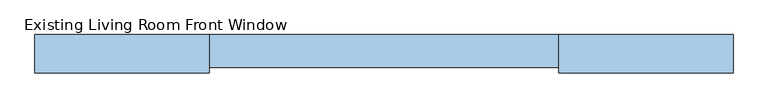
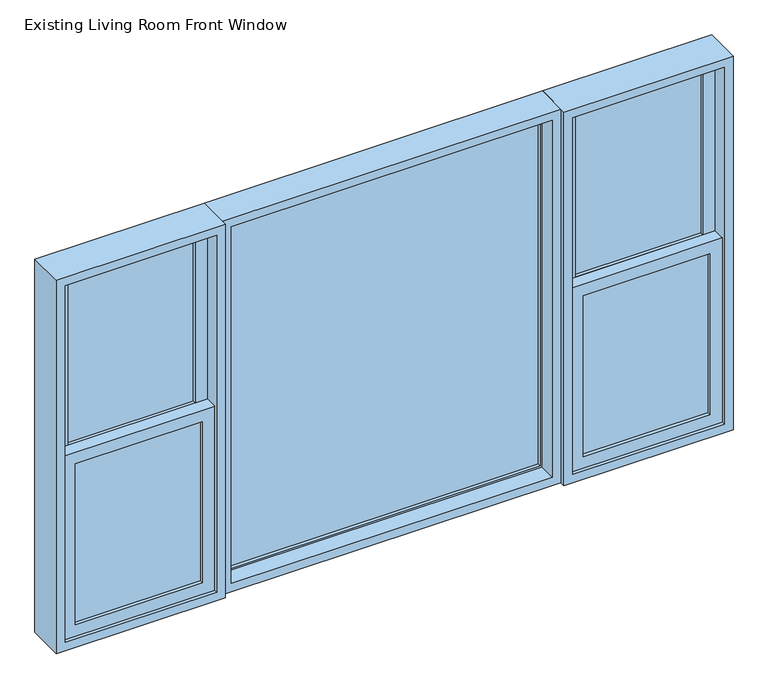
"""IFC4 building model written with IfcOpenShell, lengths in millimetres: window geometry, Existing Living Room Front Window."""

from ifc_helpers import new_model, si_unit, frame, origin, place, context, project, spatial, polyline, outline, extrude, faceted_brep, source, transform, mapped, element, save


def existing_living_room_front_window_f3d2da23(model_context):
    return source(origin(), model_context, "Body", "SolidModel", [
        extrude(outline(polyline([(-1143.0, 82.55), (-685.8, 82.55), (-685.8, 76.2), (-1143.0, 76.2), (-1143.0, 82.55)])), frame((0.0, 0.0, 990.6), z_axis=(0.0, 0.0, 1.0), x_axis=(1.0, 0.0, 0.0)), (0.0, 0.0, 1.0), 612.775),
        extrude(outline(polyline([(-685.8, 69.85), (-685.8, 63.5), (-1143.0, 63.5), (-1143.0, 69.85), (-685.8, 69.85)])), frame((0.0, 0.0, 990.6), z_axis=(0.0, 0.0, 1.0), x_axis=(1.0, 0.0, 0.0)), (0.0, 0.0, 1.0), 612.775),
        extrude(outline(polyline([(-1143.0, 127.0), (-685.8, 127.0), (-685.8, 120.65), (-1143.0, 120.65), (-1143.0, 127.0)])), frame((0.0, 0.0, 1647.825), z_axis=(0.0, 0.0, 1.0), x_axis=(1.0, 0.0, 0.0)), (0.0, 0.0, 1.0), 612.775),
        extrude(outline(polyline([(-685.8, 114.3), (-685.8, 107.95), (-1143.0, 107.95), (-1143.0, 114.3), (-685.8, 114.3)])), frame((0.0, 0.0, 1647.825), z_axis=(0.0, 0.0, 1.0), x_axis=(1.0, 0.0, 0.0)), (0.0, 0.0, 1.0), 612.775),
        extrude(outline(polyline([(1647.825, -641.35), (1647.825, -1187.45), (946.15, -1187.45), (946.15, -641.35), (1647.825, -641.35)]), holes=[polyline([(1603.375, -1143.0), (1603.375, -685.8), (990.6, -685.8), (990.6, -1143.0), (1603.375, -1143.0)])]), frame((0.0, 50.8, 0.0), z_axis=(0.0, 1.0, 0.0), x_axis=(0.0, 0.0, 1.0)), (0.0, 0.0, 1.0), 44.45),
        extrude(outline(polyline([(2305.05, -641.35), (2305.05, -1187.45), (1603.375, -1187.45), (1603.375, -641.35), (2305.05, -641.35)]), holes=[polyline([(2260.6, -1143.0), (2260.6, -685.8), (1647.825, -685.8), (1647.825, -1143.0), (2260.6, -1143.0)])]), frame((0.0, 95.25, 0.0), z_axis=(0.0, 1.0, 0.0), x_axis=(0.0, 0.0, 1.0)), (0.0, 0.0, 1.0), 44.45),
        extrude(outline(polyline([(2336.8, -609.6), (2336.8, -1219.2), (914.4, -1219.2), (914.4, -609.6), (2336.8, -609.6)]), holes=[polyline([(2305.05, -1187.45), (2305.05, -641.35), (946.15, -641.35), (946.15, -1187.45), (2305.05, -1187.45)])]), frame((0.0, 38.1, 0.0), z_axis=(0.0, 1.0, 0.0), x_axis=(0.0, 0.0, 1.0)), (0.0, 0.0, 1.0), 133.35),
        extrude(outline(polyline([(685.8, 82.55), (1143.0, 82.55), (1143.0, 76.2), (685.8, 76.2), (685.8, 82.55)])), frame((0.0, 0.0, 990.6), z_axis=(0.0, 0.0, 1.0), x_axis=(1.0, 0.0, 0.0)), (0.0, 0.0, 1.0), 612.775),
        extrude(outline(polyline([(1143.0, 69.85), (1143.0, 63.5), (685.8, 63.5), (685.8, 69.85), (1143.0, 69.85)])), frame((0.0, 0.0, 990.6), z_axis=(0.0, 0.0, 1.0), x_axis=(1.0, 0.0, 0.0)), (0.0, 0.0, 1.0), 612.775),
        extrude(outline(polyline([(685.8, 127.0), (1143.0, 127.0), (1143.0, 120.65), (685.8, 120.65), (685.8, 127.0)])), frame((0.0, 0.0, 1647.825), z_axis=(0.0, 0.0, 1.0), x_axis=(1.0, 0.0, 0.0)), (0.0, 0.0, 1.0), 612.775),
        extrude(outline(polyline([(1143.0, 114.3), (1143.0, 107.95), (685.8, 107.95), (685.8, 114.3), (1143.0, 114.3)])), frame((0.0, 0.0, 1647.825), z_axis=(0.0, 0.0, 1.0), x_axis=(1.0, 0.0, 0.0)), (0.0, 0.0, 1.0), 612.775),
        extrude(outline(polyline([(1647.825, 1187.45), (1647.825, 641.35), (946.15, 641.35), (946.15, 1187.45), (1647.825, 1187.45)]), holes=[polyline([(1603.375, 685.8), (1603.375, 1143.0), (990.6, 1143.0), (990.6, 685.8), (1603.375, 685.8)])]), frame((0.0, 50.8, 0.0), z_axis=(0.0, 1.0, 0.0), x_axis=(0.0, 0.0, 1.0)), (0.0, 0.0, 1.0), 44.45),
        extrude(outline(polyline([(2305.05, 1187.45), (2305.05, 641.35), (1603.375, 641.35), (1603.375, 1187.45), (2305.05, 1187.45)]), holes=[polyline([(2260.6, 685.8), (2260.6, 1143.0), (1647.825, 1143.0), (1647.825, 685.8), (2260.6, 685.8)])]), frame((0.0, 95.25, 0.0), z_axis=(0.0, 1.0, 0.0), x_axis=(0.0, 0.0, 1.0)), (0.0, 0.0, 1.0), 44.45),
        extrude(outline(polyline([(2336.8, 1219.2), (2336.8, 609.6), (914.4, 609.6), (914.4, 1219.2), (2336.8, 1219.2)]), holes=[polyline([(2305.05, 641.35), (2305.05, 1187.45), (946.15, 1187.45), (946.15, 641.35), (2305.05, 641.35)])]), frame((0.0, 38.1, 0.0), z_axis=(0.0, 1.0, 0.0), x_axis=(0.0, 0.0, 1.0)), (0.0, 0.0, 1.0), 133.35),
        extrude(outline(polyline([(-571.5, 152.4), (571.5, 152.4), (571.5, 146.05), (-571.5, 146.05), (-571.5, 152.4)])), frame((0.0, 0.0, 952.5), z_axis=(0.0, 0.0, 1.0), x_axis=(1.0, 0.0, 0.0)), (0.0, 0.0, 1.0), 1346.2),
        extrude(outline(polyline([(571.5, 133.35), (-571.5, 133.35), (-571.5, 139.7), (571.5, 139.7), (571.5, 133.35)])), frame((0.0, 0.0, 952.5), z_axis=(0.0, 0.0, 1.0), x_axis=(1.0, 0.0, 0.0)), (0.0, 0.0, 1.0), 1346.2),
        extrude(outline(polyline([(927.1, -596.9), (927.1, 596.9), (2324.1, 596.9), (2324.1, -596.9), (927.1, -596.9)]), holes=[polyline([(952.5, 571.5), (952.5, -571.5), (2298.7, -571.5), (2298.7, 571.5), (952.5, 571.5)])]), frame((0.0, 120.65, 0.0), z_axis=(0.0, 1.0, 0.0), x_axis=(0.0, 0.0, 1.0)), (0.0, 0.0, 1.0), 44.45),
        faceted_brep([(-609.6, 57.15, 2336.8), (609.6, 57.15, 2336.8), (609.6, 171.45, 2336.8), (-609.6, 171.45, 2336.8), (609.6, 57.15, 914.4), (609.6, 171.45, 914.4), (-609.6, 57.15, 914.4), (-609.6, 171.45, 914.4), (-577.85, 57.15, 2305.05), (577.85, 57.15, 2305.05), (577.85, 57.15, 946.15), (-577.85, 57.15, 946.15), (596.9, 171.45, 2324.1), (-596.9, 171.45, 2324.1), (-596.9, 171.45, 927.1), (596.9, 171.45, 927.1), (-577.85, 120.65, 2305.05), (577.85, 120.65, 2305.05), (596.9, 120.65, 2324.1), (-596.9, 120.65, 2324.1), (577.85, 120.65, 946.15), (596.9, 120.65, 927.1), (-577.85, 120.65, 946.15), (-596.9, 120.65, 927.1)], [[[0, 1, 2, 3]], [[1, 4, 5, 2]], [[4, 6, 7, 5]], [[1, 0, 6, 4], [8, 9, 10, 11]], [[6, 0, 3, 7]], [[3, 2, 5, 7], [12, 13, 14, 15]], [[16, 17, 9, 8]], [[13, 12, 18, 19]], [[17, 20, 10, 9]], [[12, 15, 21, 18]], [[20, 22, 11, 10]], [[15, 14, 23, 21]], [[22, 16, 8, 11]], [[19, 18, 21, 23], [17, 16, 22, 20]], [[14, 13, 19, 23]]]),
    ])


if __name__ == "__main__":
    model = new_model("IFC4")
    model_context = context("Model", 3, world=origin())
    ifc_project = project(units=[si_unit("LENGTHUNIT", "METRE", prefix="MILLI")], contexts=[model_context])
    site = spatial("IfcSite", under=ifc_project)
    building = spatial("IfcBuilding", under=site)
    placement = place(None, origin())
    existing_living_room_front_window_shape = existing_living_room_front_window_f3d2da23(model_context)
    element("IfcWindow", 1, ObjectType="Existing Living Room Front Window : (2) 2'-0\" x 4'-8\" DH + 4'-0\" x 4'-8\" FX", at=placement, inside=building, context=model_context, shape_type="MappedRepresentation", body=[
        mapped(existing_living_room_front_window_shape, transform((0.0, 0.0, 0.0), x_axis=(1.0, 0.0, 0.0), y_axis=(0.0, 1.0, 0.0), z_axis=(0.0, 0.0, 1.0))),
    ])
    save(model, "model.ifc")

# Revit data of these elements
# Type "Existing Living Room Front Window : (2) 2'-0\" x 4'-8\" DH + 4'-0\" x 4'-8\" FX"
#   Type Mark = "21"
#   Analytic Construction = "<None>"
#   Window Inset = 0' - 0 3/4"
#   Side Window Width = 2' - 0"
#   Side Window Location = 2' - 0"
#   Middle Window Width = 4' - 0"
#   Height = 4' - 8"
#   Default Sill Height = 3' - 0"
#   Width = 8' - 0"
#   Top Muntin Visibility = yes
#   Side Window Nested Trim Visibility = no
#   Interior Trim Visibility [instance default] = yes
#   Fixed Muntin Visibility = no
#   Exterior Trim Visibility [instance default] = yes
#   Define Thermal Properties by = 1
#   Bottom Muntin Visibility = yes
#   Sash Material = Sash
#   Right Side Window Type = element 472097
#   Left Side Window Type = element 472097
#   Interior Trim = Trim-Window-Interior-Flat : Picture Frame
#   Interior Trim Material = Wood - Stained
#   Interior Frame Material = Wood - Stained
#   Glass Pane Material = Glass
#   Exterior Trim Material = Clad - White
#   Exterior Trim = Trim-Window-Exterior-Flat : with Sill
#   Exterior Frame Material = Clad - White
#   Rough Width = 0
#   Rough Height = 0
#   Wall Closure = (empty or 0)
# Element 1 (IfcWindow, "Existing Living Room Front Window : (2) 2'-0\" x 4'-8\" DH + 4'-0\" x 4'-8\" FX")
#   Materials on its faces: "Wood - Stained", "Glass", "Clad - White"
# Materials
#   "Sash": class "Wood", colour RGB 224 178 126, transparency 0, Cost = 0
#   "Wood - Stained": class "Wood", colour RGB 224 178 126, transparency 0, Cost = 0
#   "Glass": class "Glass", colour RGB 0 128 192, transparency 0.75, Description = "Soda Lime Glass", Cost = 0
#   "Clad - White": class "Wood", colour RGB 245 245 243, transparency 0, Cost = 0
